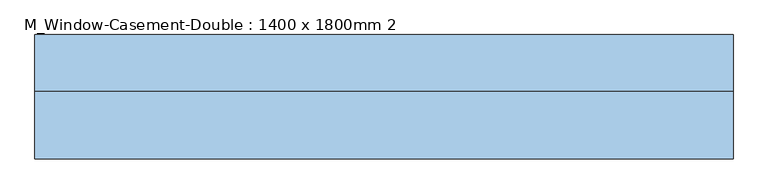
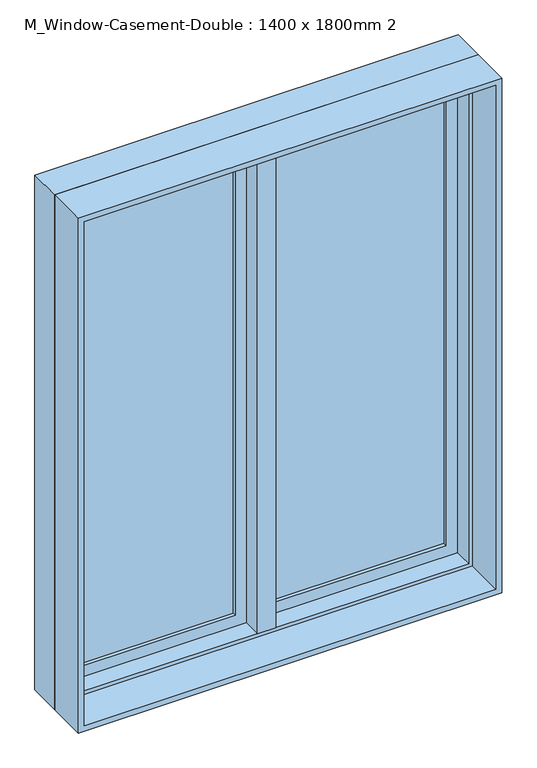
"""IFC4 building model written with IfcOpenShell, lengths in millimetres: window geometry, M_Window-Casement-Double : 1400 x 1800mm 2."""

import ifcopenshell
import ifcopenshell.guid

model = None  # the IFC model being written
_history = None  # IfcOwnerHistory: only IFC2X3 demands one
_inside = {}  # id of a spatial element -> (the spatial element, [elements in it])
_under = {}  # id of a project, library or spatial element -> (it, [spatial elements below it])
_declared = {}  # id of a project -> (the project, [libraries it declares])
_typed = {}  # id of a type object -> (the type object, [elements of that type])
_made_of = {}  # id of a material, layer set ... -> (it, [elements and type objects made of it])


def new_model(schema):
    """Start an empty IFC model of exactly this schema.

    Asked for "IFC4X3", IfcOpenShell would pick the latest addendum, in which some entities
    have other attributes; the version numbers below select the first issue.
    IFC2X3 requires an IfcOwnerHistory on every rooted entity: one is made here for all.
    """
    global model, _history
    if schema == "IFC4X3":
        model = ifcopenshell.file(schema_version=(4, 3, 0, 0))
    else:
        model = ifcopenshell.file(schema=schema)
    _inside.clear()
    _under.clear()
    _declared.clear()
    _typed.clear()
    _made_of.clear()
    _history = None
    if model.schema == "IFC2X3":
        org = make("IfcOrganization", Name="unknown")
        user = make(
            "IfcPersonAndOrganization",
            ThePerson=make("IfcPerson", FamilyName="unknown"),
            TheOrganization=org,
        )
        app = make(
            "IfcApplication",
            ApplicationDeveloper=org,
            Version="unknown",
            ApplicationFullName="unknown",
            ApplicationIdentifier="unknown",
        )
        _history = make(
            "IfcOwnerHistory",
            OwningUser=user,
            OwningApplication=app,
            ChangeAction="ADDED",
            CreationDate=0,
        )
    return model


def make(cls, **values):
    """One entity of the class cls with the attributes given. An attribute that is None is left unset."""
    return model.create_entity(
        cls, **{name: value for name, value in values.items() if value is not None}
    )


def rooted(cls, **values):
    """An entity with a GlobalId (a new one), such as an element, a storey or a relation."""
    return make(cls, GlobalId=ifcopenshell.guid.new(), OwnerHistory=_history, **values)


def si_unit(unit_type, name, prefix=None):
    """IfcSIUnit, for example si_unit("LENGTHUNIT", "METRE", prefix="MILLI")."""
    return make("IfcSIUnit", UnitType=unit_type, Prefix=prefix, Name=name)


def assignment(units):
    """IfcUnitAssignment: the units of a project."""
    return None if units is None else make("IfcUnitAssignment", Units=units)


def point(xyz):
    """IfcCartesianPoint."""
    return None if xyz is None else make("IfcCartesianPoint", Coordinates=xyz)


def direction(xyz):
    """IfcDirection."""
    return None if xyz is None else make("IfcDirection", DirectionRatios=xyz)


def frame(location, z_axis=None, x_axis=None):
    """IfcAxis2Placement3D, a coordinate frame: its origin and axes. An axis left out is left unset."""
    return make(
        "IfcAxis2Placement3D",
        Location=point(location),
        Axis=direction(z_axis),
        RefDirection=direction(x_axis),
    )


def origin():
    """The frame at (0, 0, 0) with its axes left unset."""
    return frame((0.0, 0.0, 0.0))


def place(relative_to, where):
    """IfcLocalPlacement: puts the frame where relative to a parent placement (None: the world)."""
    return make(
        "IfcLocalPlacement", PlacementRelTo=relative_to, RelativePlacement=where
    )


def context(
    kind, dimensions, precision=None, world=None, true_north=None, identifier=None
):
    """IfcGeometricRepresentationContext, for example the 3D "Model" context."""
    return make(
        "IfcGeometricRepresentationContext",
        ContextIdentifier=identifier,
        ContextType=kind,
        CoordinateSpaceDimension=dimensions,
        Precision=precision,
        WorldCoordinateSystem=world,
        TrueNorth=true_north,
    )


def project(units=None, contexts=None):
    """IfcProject with its units and contexts."""
    return rooted(
        "IfcProject",
        Name="project",
        RepresentationContexts=contexts,
        UnitsInContext=assignment(units),
    )


def spatial(cls, under=None, at=None, **own):
    """A site, building, storey or space (cls), placed at a placement, below another one or the project."""
    s = rooted(cls, ObjectPlacement=at, **own)
    if under is not None:
        _under.setdefault(under.id(), (under, []))[1].append(s)
    return s


def polyline(points):
    """IfcPolyline through the points."""
    return make("IfcPolyline", Points=[point(p) for p in points])


def outline(outer, holes=None, kind="AREA"):
    """IfcArbitraryClosedProfileDef: a profile drawn as a closed curve; with holes, ...WithVoids."""
    if holes is None:
        return make("IfcArbitraryClosedProfileDef", ProfileType=kind, OuterCurve=outer)
    return make(
        "IfcArbitraryProfileDefWithVoids",
        ProfileType=kind,
        OuterCurve=outer,
        InnerCurves=holes,
    )


def extrude(swept, where, along, depth):
    """IfcExtrudedAreaSolid: the profile swept, set in the frame where, extruded along a direction by depth."""
    return make(
        "IfcExtrudedAreaSolid",
        SweptArea=swept,
        Position=where,
        ExtrudedDirection=direction(along),
        Depth=depth,
    )


def faces_of(points, faces, orient=None, outer=None):
    """IfcFace entities. A face is a list of loops; a loop is a list of indices into points, from 0.

    orient and outer hold one flag for each loop. By default every Orientation is true, the
    first loop of a face is its IfcFaceOuterBound and the others are IfcFaceBound.
    """
    made = []
    for i, loops in enumerate(faces):
        bounds = []
        for j, loop in enumerate(loops):
            is_outer = j == 0 if outer is None else outer[i][j]
            bounds.append(
                make(
                    "IfcFaceOuterBound" if is_outer else "IfcFaceBound",
                    Bound=make("IfcPolyLoop", Polygon=[points[k] for k in loop]),
                    Orientation=True if orient is None else orient[i][j],
                )
            )
        made.append(make("IfcFace", Bounds=bounds))
    return made


def faceted_brep(points, faces, orient=None, outer=None, voids=None):
    """IfcFacetedBrep: a solid bounded by flat faces; with voids (closed shells), ...WithVoids."""
    shared = [point(p) for p in points]
    hull = make("IfcClosedShell", CfsFaces=faces_of(shared, faces, orient, outer))
    if voids is None:
        return make("IfcFacetedBrep", Outer=hull)
    return make(
        "IfcFacetedBrepWithVoids",
        Outer=hull,
        Voids=[
            make(cls, CfsFaces=faces_of(shared, fs, o, b)) for cls, fs, o, b in voids
        ],
    )


def shape(context_of_items, identifier, shape_type, items):
    """IfcShapeRepresentation: the items that make up one representation, for example the "Body"."""
    return make(
        "IfcShapeRepresentation",
        ContextOfItems=context_of_items,
        RepresentationIdentifier=identifier,
        RepresentationType=shape_type,
        Items=items,
    )


def source(mapping_origin, context_of_items, identifier, shape_type, items):
    """IfcRepresentationMap: a shape defined once, which mapped items show again and again."""
    return make(
        "IfcRepresentationMap",
        MappingOrigin=mapping_origin,
        MappedRepresentation=shape(context_of_items, identifier, shape_type, items),
    )


def transform(
    local_origin,
    x_axis=None,
    y_axis=None,
    z_axis=None,
    scale=None,
    scale2=None,
    scale3=None,
    uniform=True,
):
    """IfcCartesianTransformationOperator3D, or its non-uniform kind. x_axis, y_axis, z_axis: its Axis1, 2, 3."""
    if uniform:
        return make(
            "IfcCartesianTransformationOperator3D",
            Axis1=direction(x_axis),
            Axis2=direction(y_axis),
            LocalOrigin=point(local_origin),
            Scale=scale,
            Axis3=direction(z_axis),
        )
    return make(
        "IfcCartesianTransformationOperator3DnonUniform",
        Axis1=direction(x_axis),
        Axis2=direction(y_axis),
        LocalOrigin=point(local_origin),
        Scale=scale,
        Axis3=direction(z_axis),
        Scale2=scale2,
        Scale3=scale3,
    )


def mapped(mapping_source, mapping_target):
    """IfcMappedItem: shows the shape of a source again, moved by a transform."""
    return make(
        "IfcMappedItem", MappingSource=mapping_source, MappingTarget=mapping_target
    )


def made_of(thing, what):
    """Note that an element or type object is made of a material, layer set ...; save() writes the relation."""
    if what is not None:
        _made_of.setdefault(what.id(), (what, []))[1].append(thing)
    return thing


def element(
    cls,
    number,
    at=None,
    inside=None,
    cuts=None,
    type_object=None,
    material=None,
    context=None,
    identifier="Body",
    shape_type=None,
    held_by="IfcProductDefinitionShape",
    body=None,
    shapes=None,
    **own,
):
    """One element of the class cls, such as IfcWall. Its Tag is "e" and its number.

    at: its placement. inside: the storey or other place that contains it. cuts: it is an
    opening in that element (IfcRelVoidsElement). A single representation is given by context,
    identifier, shape_type and body (its items); several are given by shapes. held_by: the class
    of the entity that holds the representations. save() writes the other relations.
    """
    e = rooted(cls, Tag="e%d" % number, ObjectPlacement=at, **own)
    if body is not None:
        shapes = [shape(context, identifier, shape_type, body)]
    if shapes is not None:
        e.Representation = make(held_by, Representations=shapes)
    if inside is not None:
        _inside.setdefault(inside.id(), (inside, []))[1].append(e)
    if cuts is not None:
        rooted(
            "IfcRelVoidsElement", RelatingBuildingElement=cuts, RelatedOpeningElement=e
        )
    if type_object is not None:
        _typed.setdefault(type_object.id(), (type_object, []))[1].append(e)
    return made_of(e, material)


def aggregate(whole, parts):
    """IfcRelAggregates: a whole, such as a stair, and the parts it consists of."""
    return rooted("IfcRelAggregates", RelatingObject=whole, RelatedObjects=parts)


def save(model, path):
    """Write the relations noted so far, then the file.

    IfcRelAggregates (storeys below a building ...), IfcRelContainedInSpatialStructure (elements
    in a storey), IfcRelDefinesByType, IfcRelAssociatesMaterial and IfcRelDeclares: one each for
    every whole, place, type object, material and project.
    """
    for whole, parts in _under.values():
        aggregate(whole, parts)
    for where, things in _inside.values():
        rooted(
            "IfcRelContainedInSpatialStructure",
            RelatedElements=things,
            RelatingStructure=where,
        )
    for kind, things in _typed.values():
        rooted("IfcRelDefinesByType", RelatedObjects=things, RelatingType=kind)
    for what, things in _made_of.values():
        rooted("IfcRelAssociatesMaterial", RelatedObjects=things, RelatingMaterial=what)
    for by, libraries in _declared.values():
        rooted("IfcRelDeclares", RelatingContext=by, RelatedDefinitions=libraries)
    model.write(path)


def m_window_casement_double_1400_x_1800mm_2_db642eaa(model_context):
    return source(origin(), model_context, "Body", "SolidModel", [
        faceted_brep([(9.525, 134.05, 2387.3), (-9.525, 134.05, 2387.3), (-9.525, 83.25, 2387.3), (9.525, 83.25, 2387.3), (9.525, 134.05, 612.7), (9.525, 83.25, 612.7), (-9.525, 83.25, 612.7), (-9.525, 134.05, 612.7), (-9.525, 83.25, 631.75), (-9.525, 83.25, 2368.25), (-30.1625, 83.25, 631.75), (-30.1625, 83.25, 2368.25), (-30.1625, 19.75, 631.75), (-30.1625, 19.75, 2368.25), (30.1625, 19.75, 631.75), (30.1625, 19.75, 2368.25), (30.1625, 83.25, 631.75), (30.1625, 83.25, 2368.25), (9.525, 83.25, 631.75), (9.525, 83.25, 2368.25)], [[[0, 1, 2, 3]], [[4, 5, 6, 7]], [[1, 0, 4, 7]], [[2, 1, 7, 6, 8, 9]], [[9, 8, 10, 11]], [[11, 10, 12, 13]], [[13, 12, 14, 15]], [[15, 14, 16, 17]], [[17, 16, 18, 19]], [[0, 3, 19, 18, 5, 4]], [[18, 8, 6, 5]], [[9, 19, 3, 2]], [[8, 18, 16, 14, 12, 10]], [[19, 9, 11, 13, 15, 17]]]),
        extrude(outline(polyline([(-66.675, 115.0), (-66.675, 108.65), (-630.15, 108.65), (-630.15, 115.0), (-66.675, 115.0)])), frame((0.0, 0.0, 669.85), z_axis=(0.0, 0.0, 1.0), x_axis=(1.0, 0.0, 0.0)), (0.0, 0.0, 1.0), 1660.3),
        extrude(outline(polyline([(-630.15, 95.95), (-630.15, 102.3), (-66.675, 102.3), (-66.675, 95.95), (-630.15, 95.95)])), frame((0.0, 0.0, 669.85), z_axis=(0.0, 0.0, 1.0), x_axis=(1.0, 0.0, 0.0)), (0.0, 0.0, 1.0), 1660.3),
        extrude(outline(polyline([(630.15, 115.0), (630.15, 108.65), (66.675, 108.65), (66.675, 115.0), (630.15, 115.0)])), frame((0.0, 0.0, 669.85), z_axis=(0.0, 0.0, 1.0), x_axis=(1.0, 0.0, 0.0)), (0.0, 0.0, 1.0), 1660.3),
        extrude(outline(polyline([(66.675, 95.95), (66.675, 102.3), (630.15, 102.3), (630.15, 95.95), (66.675, 95.95)])), frame((0.0, 0.0, 669.85), z_axis=(0.0, 0.0, 1.0), x_axis=(1.0, 0.0, 0.0)), (0.0, 0.0, 1.0), 1660.3),
        extrude(outline(polyline([(2387.3, -687.3), (612.7, -687.3), (612.7, -9.525), (2387.3, -9.525), (2387.3, -687.3)]), holes=[polyline([(2330.15, -66.675), (669.85, -66.675), (669.85, -630.15), (2330.15, -630.15), (2330.15, -66.675)])]), frame((0.0, 83.25, 0.0), z_axis=(0.0, 1.0, 0.0), x_axis=(0.0, 0.0, 1.0)), (0.0, 0.0, 1.0), 44.45),
        extrude(outline(polyline([(612.7, 687.3), (2387.3, 687.3), (2387.3, 9.525), (612.7, 9.525), (612.7, 687.3)]), holes=[polyline([(669.85, 66.675), (2330.15, 66.675), (2330.15, 630.15), (669.85, 630.15), (669.85, 66.675)])]), frame((0.0, 83.25, 0.0), z_axis=(0.0, 1.0, 0.0), x_axis=(0.0, 0.0, 1.0)), (0.0, 0.0, 1.0), 44.45),
        extrude(outline(polyline([(2400.0, -700.0), (600.0, -700.0), (600.0, 700.0), (2400.0, 700.0), (2400.0, -700.0)]), holes=[polyline([(2380.95, 680.95), (619.05, 680.95), (619.05, -680.95), (2380.95, -680.95), (2380.95, 680.95)])]), frame((0.0, -115.0, 0.0), z_axis=(0.0, 1.0, 0.0), x_axis=(0.0, 0.0, 1.0)), (0.0, 0.0, 1.0), 134.75),
        faceted_brep([(668.25, 83.25, 2368.25), (668.25, 19.75, 2368.25), (-668.25, 19.75, 2368.25), (-668.25, 83.25, 2368.25), (687.3, 134.05, 2387.3), (687.3, 83.25, 2387.3), (-687.3, 83.25, 2387.3), (-687.3, 134.05, 2387.3), (700.0, 19.75, 2400.0), (700.0, 134.05, 2400.0), (-700.0, 134.05, 2400.0), (-700.0, 19.75, 2400.0), (-668.25, 19.75, 631.75), (-668.25, 83.25, 631.75), (-687.3, 83.25, 612.7), (-687.3, 134.05, 612.7), (-700.0, 134.05, 600.0), (-700.0, 19.75, 600.0), (668.25, 19.75, 631.75), (668.25, 83.25, 631.75), (687.3, 83.25, 612.7), (687.3, 134.05, 612.7), (700.0, 134.05, 600.0), (700.0, 19.75, 600.0)], [[[0, 1, 2, 3]], [[4, 5, 6, 7]], [[8, 9, 10, 11]], [[3, 2, 12, 13]], [[7, 6, 14, 15]], [[11, 10, 16, 17]], [[13, 12, 18, 19]], [[15, 14, 20, 21]], [[17, 16, 22, 23]], [[11, 17, 23, 8], [1, 18, 12, 2]], [[19, 18, 1, 0]], [[5, 20, 14, 6], [3, 13, 19, 0]], [[21, 20, 5, 4]], [[23, 22, 9, 8]], [[9, 22, 16, 10], [7, 15, 21, 4]]]),
    ])


if __name__ == "__main__":
    model = new_model("IFC4")
    model_context = context("Model", 3, world=origin())
    ifc_project = project(units=[si_unit("LENGTHUNIT", "METRE", prefix="MILLI")], contexts=[model_context])
    site = spatial("IfcSite", under=ifc_project)
    building = spatial("IfcBuilding", under=site)
    placement = place(None, origin())
    m_window_casement_double_1400_x_1800mm_2_shape = m_window_casement_double_1400_x_1800mm_2_db642eaa(model_context)
    element("IfcWindow", 1, ObjectType="M_Window-Casement-Double : 1400 x 1800mm 2", at=placement, inside=building, context=model_context, shape_type="MappedRepresentation", body=[
        mapped(m_window_casement_double_1400_x_1800mm_2_shape, transform((0.0, 0.0, 0.0), x_axis=(1.0, 0.0, 0.0), y_axis=(0.0, 1.0, 0.0), z_axis=(0.0, 0.0, 1.0))),
    ])
    save(model, "model.ifc")

# Revit data of these elements
# Type "M_Window-Casement-Double : 1400 x 1800mm 2"
#   Type Mark = "27"
#   Fire Rating = "0.5h"
#   Assembly Code = "B2020100"
#   Analytic Construction = "Double glazing - domestic"
#   Frame Extension [instance default] = 0.635 cm
#   Window Inset [instance default] = 0 cm
#   Wall Thickness [instance default] = 15 cm
#   Interior Wall Closure [instance default] = 5.475 cm
#   Half Width = 70 cm
#   Visual Light Transmittance = 0.81
#   Thermal Resistance (R) = 0.319569 (m²·K)/W
#   Solar Heat Gain Coefficient = 0.76
#   Rough Width = 141.5 cm
#   Rough Height = 181.5 cm
#   Height = 180 cm
#   Heat Transfer Coefficient (U) = 3.12929 W/(m²·K)
#   Exterior Wall Closure [instance default] = 3.18 cm
#   Extension Jamb [instance default] = 5.475 cm
#   Default Sill Height = 60 cm
#   Width = 140 cm
#   Muntin Visibility = yes
#   Interior Trim Visibility [instance default] = yes
#   Exterior Trim Visibility [instance default] = yes
#   Extension Jamb Visibility [instance default] = yes
#   Interior Trim Material = Wood - Stained
#   Muntin Pattern = M_Muntin Pattern_2x2 : M_Muntin Pattern_2x2
#   Interior Trim = M_Trim-Window-Interior-Flat : Picture Frame
#   Interior Frame Material = Wood - Stained
#   Glass Panel Material = Glass
#   Exterior Trim Material = Clad - White
#   Exterior Trim = M_Trim-Window-Exterior-Flat : with Sill
#   Exterior Frame Material = Clad - White
#   Wall Closure = (empty or 0)
# Element 1 (IfcWindow, "M_Window-Casement-Double : 1400 x 1800mm 2")
#   Wall Thickness = 23 cm
#   Extension Jamb = 13.475 cm
#   Materials on its faces: "Wood - Stained", "Glass", "Clad - White"
# Materials
#   "Wood - Stained": class "Wood", colour RGB 224 178 126, transparency 0, Cost = 0
#   "Glass": class "Glass", colour RGB 0 128 192, transparency 0.9, Description = "Soda Lime Glass", Cost = 0
#   "Clad - White": class "Wood", colour RGB 242 242 238, transparency 0, Cost = 0
